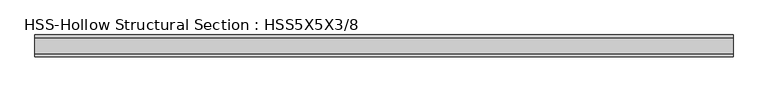
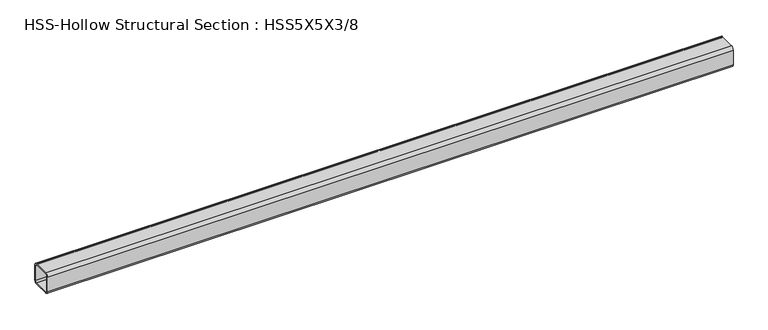
"""IFC4 building model written with IfcOpenShell, lengths in millimetres: member geometry, HSS-Hollow Structural Section : HSS5X5X3/8."""

from ifc_helpers import new_model, si_unit, point, frame, frame_2d, origin, place, context, project, spatial, polyline, circle_curve, trimmed, segment, composite_curve, outline, extrude, source, transform, mapped, element, save


def hss_hollow_structural_section_hss5x5x3_8_d39f42fe(model_context):
    return source(origin(), model_context, "Body", "SweptSolid", [
        extrude(outline(composite_curve([segment(polyline([(63.5, 45.7708), (63.5, -45.7708)]), True, "CONTINUOUS"), segment(trimmed(circle_curve(frame_2d((45.7708, -45.7708)), 17.7292), [point((63.5, -45.7708))], [point((45.7708, -63.5))], False, "CARTESIAN"), True, "CONTINUOUS"), segment(polyline([(45.7708, -63.5), (-45.7708, -63.5)]), True, "CONTINUOUS"), segment(trimmed(circle_curve(frame_2d((-45.7708, -45.7708)), 17.7292), [point((-45.7708, -63.5))], [point((-63.5, -45.7708))], False, "CARTESIAN"), True, "CONTINUOUS"), segment(polyline([(-63.5, -45.7708), (-63.5, 45.7708)]), True, "CONTINUOUS"), segment(trimmed(circle_curve(frame_2d((-45.7708, 45.7708)), 17.7292), [point((-63.5, 45.7708))], [point((-45.7708, 63.5))], False, "CARTESIAN"), True, "CONTINUOUS"), segment(polyline([(-45.7708, 63.5), (45.7708, 63.5)]), True, "CONTINUOUS"), segment(trimmed(circle_curve(frame_2d((45.7708, 45.7708)), 17.7292), [point((45.7708, 63.5))], [point((63.5, 45.7708))], False, "CARTESIAN"), True, "CONTINUOUS")], self_intersect=False), holes=[composite_curve([segment(trimmed(circle_curve(frame_2d((-45.7708, 45.7708)), 8.8646), [point((-45.7708, 54.6354))], [point((-54.6354, 45.7708))], True, "CARTESIAN"), True, "CONTINUOUS"), segment(polyline([(-54.6354, 45.7708), (-54.6354, -45.7708)]), True, "CONTINUOUS"), segment(trimmed(circle_curve(frame_2d((-45.7708, -45.7708)), 8.8646), [point((-54.6354, -45.7708))], [point((-45.7708, -54.6354))], True, "CARTESIAN"), True, "CONTINUOUS"), segment(polyline([(-45.7708, -54.6354), (45.7708, -54.6354)]), True, "CONTINUOUS"), segment(trimmed(circle_curve(frame_2d((45.7708, -45.7708)), 8.8646), [point((45.7708, -54.6354))], [point((54.6354, -45.7708))], True, "CARTESIAN"), True, "CONTINUOUS"), segment(polyline([(54.6354, -45.7708), (54.6354, 45.7708)]), True, "CONTINUOUS"), segment(trimmed(circle_curve(frame_2d((45.7708, 45.7708)), 8.8646), [point((54.6354, 45.7708))], [point((45.7708, 54.6354))], True, "CARTESIAN"), True, "CONTINUOUS"), segment(polyline([(45.7708, 54.6354), (-45.7708, 54.6354)]), True, "CONTINUOUS")], self_intersect=False)]), frame((-2022.2115003, 0.0, 0.0), z_axis=(1.0, 0.0, 0.0), x_axis=(0.0, 1.0, 0.0)), (0.0, 0.0, 1.0), 4044.4230006),
    ])


if __name__ == "__main__":
    model = new_model("IFC4")
    model_context = context("Model", 3, world=origin())
    ifc_project = project(units=[si_unit("LENGTHUNIT", "METRE", prefix="MILLI")], contexts=[model_context])
    site = spatial("IfcSite", under=ifc_project)
    building = spatial("IfcBuilding", under=site)
    placement = place(None, origin())
    hss_hollow_structural_section_hss5x5x3_8_shape = hss_hollow_structural_section_hss5x5x3_8_d39f42fe(model_context)
    element("IfcMember", 1, ObjectType="HSS-Hollow Structural Section : HSS5X5X3/8", at=placement, inside=building, context=model_context, shape_type="MappedRepresentation", body=[
        mapped(hss_hollow_structural_section_hss5x5x3_8_shape, transform((0.0, 0.0, 0.0), x_axis=(1.0, 0.0, 0.0), y_axis=(0.0, 1.0, 0.0), z_axis=(0.0, 0.0, 1.0))),
    ])
    save(model, "model.ifc")

# Revit data of these elements
# Type "HSS-Hollow Structural Section : HSS5X5X3/8"
#   Assembly Code = "B10"
#   Shape = "Square"
#   W = 22.3
#   Ht = 0' - 5"
#   Length [instance default] = 5' - 0"
#   b = 0' - 5"
#   kr = 0' - 0.698"
#   t = 0' - 0.349"
#   A = 0.0429167 SF
#   Structural Material [instance default] = Steel ASTM A500, Grade B, Rectangular and Square
# Element 1 (IfcMember, "HSS-Hollow Structural Section : HSS5X5X3/8")
#   Materials on its faces: "Steel ASTM A500, Grade B, Rectangular and Square"
# Materials
#   "Steel ASTM A500, Grade B, Rectangular and Square": class "Metal", colour RGB 199 199 199, transparency 0, Description = "Carbon steel", Cost = 0
